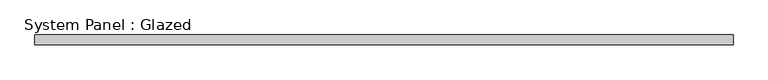
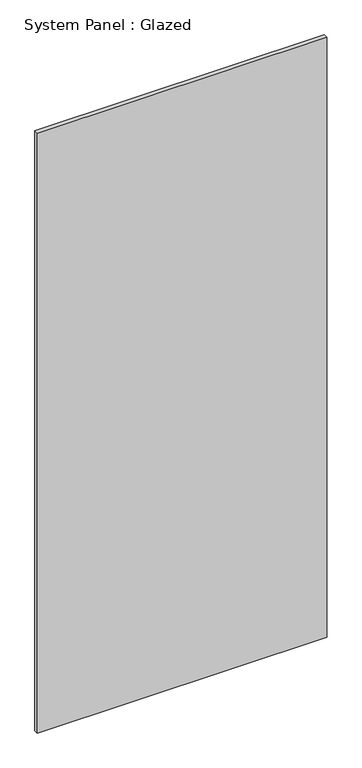
"""IFC4 building model written with IfcOpenShell, lengths in millimetres: plate geometry, System Panel : Glazed."""

import ifcopenshell
import ifcopenshell.guid

model = None  # the IFC model being written
_history = None  # IfcOwnerHistory: only IFC2X3 demands one
_inside = {}  # id of a spatial element -> (the spatial element, [elements in it])
_under = {}  # id of a project, library or spatial element -> (it, [spatial elements below it])
_declared = {}  # id of a project -> (the project, [libraries it declares])
_typed = {}  # id of a type object -> (the type object, [elements of that type])
_made_of = {}  # id of a material, layer set ... -> (it, [elements and type objects made of it])


def new_model(schema):
    """Start an empty IFC model of exactly this schema.

    Asked for "IFC4X3", IfcOpenShell would pick the latest addendum, in which some entities
    have other attributes; the version numbers below select the first issue.
    IFC2X3 requires an IfcOwnerHistory on every rooted entity: one is made here for all.
    """
    global model, _history
    if schema == "IFC4X3":
        model = ifcopenshell.file(schema_version=(4, 3, 0, 0))
    else:
        model = ifcopenshell.file(schema=schema)
    _inside.clear()
    _under.clear()
    _declared.clear()
    _typed.clear()
    _made_of.clear()
    _history = None
    if model.schema == "IFC2X3":
        org = make("IfcOrganization", Name="unknown")
        user = make(
            "IfcPersonAndOrganization",
            ThePerson=make("IfcPerson", FamilyName="unknown"),
            TheOrganization=org,
        )
        app = make(
            "IfcApplication",
            ApplicationDeveloper=org,
            Version="unknown",
            ApplicationFullName="unknown",
            ApplicationIdentifier="unknown",
        )
        _history = make(
            "IfcOwnerHistory",
            OwningUser=user,
            OwningApplication=app,
            ChangeAction="ADDED",
            CreationDate=0,
        )
    return model


def make(cls, **values):
    """One entity of the class cls with the attributes given. An attribute that is None is left unset."""
    return model.create_entity(
        cls, **{name: value for name, value in values.items() if value is not None}
    )


def rooted(cls, **values):
    """An entity with a GlobalId (a new one), such as an element, a storey or a relation."""
    return make(cls, GlobalId=ifcopenshell.guid.new(), OwnerHistory=_history, **values)


def si_unit(unit_type, name, prefix=None):
    """IfcSIUnit, for example si_unit("LENGTHUNIT", "METRE", prefix="MILLI")."""
    return make("IfcSIUnit", UnitType=unit_type, Prefix=prefix, Name=name)


def assignment(units):
    """IfcUnitAssignment: the units of a project."""
    return None if units is None else make("IfcUnitAssignment", Units=units)


def point(xyz):
    """IfcCartesianPoint."""
    return None if xyz is None else make("IfcCartesianPoint", Coordinates=xyz)


def direction(xyz):
    """IfcDirection."""
    return None if xyz is None else make("IfcDirection", DirectionRatios=xyz)


def frame(location, z_axis=None, x_axis=None):
    """IfcAxis2Placement3D, a coordinate frame: its origin and axes. An axis left out is left unset."""
    return make(
        "IfcAxis2Placement3D",
        Location=point(location),
        Axis=direction(z_axis),
        RefDirection=direction(x_axis),
    )


def origin():
    """The frame at (0, 0, 0) with its axes left unset."""
    return frame((0.0, 0.0, 0.0))


def origin_with_axes():
    """The frame at (0, 0, 0) with the z axis (0, 0, 1) and the x axis (1, 0, 0) written out."""
    return frame((0.0, 0.0, 0.0), z_axis=(0.0, 0.0, 1.0), x_axis=(1.0, 0.0, 0.0))


def place(relative_to, where):
    """IfcLocalPlacement: puts the frame where relative to a parent placement (None: the world)."""
    return make(
        "IfcLocalPlacement", PlacementRelTo=relative_to, RelativePlacement=where
    )


def context(
    kind, dimensions, precision=None, world=None, true_north=None, identifier=None
):
    """IfcGeometricRepresentationContext, for example the 3D "Model" context."""
    return make(
        "IfcGeometricRepresentationContext",
        ContextIdentifier=identifier,
        ContextType=kind,
        CoordinateSpaceDimension=dimensions,
        Precision=precision,
        WorldCoordinateSystem=world,
        TrueNorth=true_north,
    )


def project(units=None, contexts=None):
    """IfcProject with its units and contexts."""
    return rooted(
        "IfcProject",
        Name="project",
        RepresentationContexts=contexts,
        UnitsInContext=assignment(units),
    )


def spatial(cls, under=None, at=None, **own):
    """A site, building, storey or space (cls), placed at a placement, below another one or the project."""
    s = rooted(cls, ObjectPlacement=at, **own)
    if under is not None:
        _under.setdefault(under.id(), (under, []))[1].append(s)
    return s


def polyline(points):
    """IfcPolyline through the points."""
    return make("IfcPolyline", Points=[point(p) for p in points])


def outline(outer, holes=None, kind="AREA"):
    """IfcArbitraryClosedProfileDef: a profile drawn as a closed curve; with holes, ...WithVoids."""
    if holes is None:
        return make("IfcArbitraryClosedProfileDef", ProfileType=kind, OuterCurve=outer)
    return make(
        "IfcArbitraryProfileDefWithVoids",
        ProfileType=kind,
        OuterCurve=outer,
        InnerCurves=holes,
    )


def extrude(swept, where, along, depth):
    """IfcExtrudedAreaSolid: the profile swept, set in the frame where, extruded along a direction by depth."""
    return make(
        "IfcExtrudedAreaSolid",
        SweptArea=swept,
        Position=where,
        ExtrudedDirection=direction(along),
        Depth=depth,
    )


def shape(context_of_items, identifier, shape_type, items):
    """IfcShapeRepresentation: the items that make up one representation, for example the "Body"."""
    return make(
        "IfcShapeRepresentation",
        ContextOfItems=context_of_items,
        RepresentationIdentifier=identifier,
        RepresentationType=shape_type,
        Items=items,
    )


def source(mapping_origin, context_of_items, identifier, shape_type, items):
    """IfcRepresentationMap: a shape defined once, which mapped items show again and again."""
    return make(
        "IfcRepresentationMap",
        MappingOrigin=mapping_origin,
        MappedRepresentation=shape(context_of_items, identifier, shape_type, items),
    )


def transform(
    local_origin,
    x_axis=None,
    y_axis=None,
    z_axis=None,
    scale=None,
    scale2=None,
    scale3=None,
    uniform=True,
):
    """IfcCartesianTransformationOperator3D, or its non-uniform kind. x_axis, y_axis, z_axis: its Axis1, 2, 3."""
    if uniform:
        return make(
            "IfcCartesianTransformationOperator3D",
            Axis1=direction(x_axis),
            Axis2=direction(y_axis),
            LocalOrigin=point(local_origin),
            Scale=scale,
            Axis3=direction(z_axis),
        )
    return make(
        "IfcCartesianTransformationOperator3DnonUniform",
        Axis1=direction(x_axis),
        Axis2=direction(y_axis),
        LocalOrigin=point(local_origin),
        Scale=scale,
        Axis3=direction(z_axis),
        Scale2=scale2,
        Scale3=scale3,
    )


def mapped(mapping_source, mapping_target):
    """IfcMappedItem: shows the shape of a source again, moved by a transform."""
    return make(
        "IfcMappedItem", MappingSource=mapping_source, MappingTarget=mapping_target
    )


def made_of(thing, what):
    """Note that an element or type object is made of a material, layer set ...; save() writes the relation."""
    if what is not None:
        _made_of.setdefault(what.id(), (what, []))[1].append(thing)
    return thing


def element(
    cls,
    number,
    at=None,
    inside=None,
    cuts=None,
    type_object=None,
    material=None,
    context=None,
    identifier="Body",
    shape_type=None,
    held_by="IfcProductDefinitionShape",
    body=None,
    shapes=None,
    **own,
):
    """One element of the class cls, such as IfcWall. Its Tag is "e" and its number.

    at: its placement. inside: the storey or other place that contains it. cuts: it is an
    opening in that element (IfcRelVoidsElement). A single representation is given by context,
    identifier, shape_type and body (its items); several are given by shapes. held_by: the class
    of the entity that holds the representations. save() writes the other relations.
    """
    e = rooted(cls, Tag="e%d" % number, ObjectPlacement=at, **own)
    if body is not None:
        shapes = [shape(context, identifier, shape_type, body)]
    if shapes is not None:
        e.Representation = make(held_by, Representations=shapes)
    if inside is not None:
        _inside.setdefault(inside.id(), (inside, []))[1].append(e)
    if cuts is not None:
        rooted(
            "IfcRelVoidsElement", RelatingBuildingElement=cuts, RelatedOpeningElement=e
        )
    if type_object is not None:
        _typed.setdefault(type_object.id(), (type_object, []))[1].append(e)
    return made_of(e, material)


def aggregate(whole, parts):
    """IfcRelAggregates: a whole, such as a stair, and the parts it consists of."""
    return rooted("IfcRelAggregates", RelatingObject=whole, RelatedObjects=parts)


def save(model, path):
    """Write the relations noted so far, then the file.

    IfcRelAggregates (storeys below a building ...), IfcRelContainedInSpatialStructure (elements
    in a storey), IfcRelDefinesByType, IfcRelAssociatesMaterial and IfcRelDeclares: one each for
    every whole, place, type object, material and project.
    """
    for whole, parts in _under.values():
        aggregate(whole, parts)
    for where, things in _inside.values():
        rooted(
            "IfcRelContainedInSpatialStructure",
            RelatedElements=things,
            RelatingStructure=where,
        )
    for kind, things in _typed.values():
        rooted("IfcRelDefinesByType", RelatedObjects=things, RelatingType=kind)
    for what, things in _made_of.values():
        rooted("IfcRelAssociatesMaterial", RelatedObjects=things, RelatingMaterial=what)
    for by, libraries in _declared.values():
        rooted("IfcRelDeclares", RelatingContext=by, RelatedDefinitions=libraries)
    model.write(path)


def system_panel_glazed_26169dd8(model_context):
    return source(origin(), model_context, "Body", "SweptSolid", [
        extrude(outline(polyline([(890.0, 24.5), (-890.0, 24.5), (-890.0, 49.5), (890.0, 49.5), (890.0, 24.5)])), origin_with_axes(), (0.0, 0.0, 1.0), 3900.0),
    ])


if __name__ == "__main__":
    model = new_model("IFC4")
    model_context = context("Model", 3, world=origin())
    ifc_project = project(units=[si_unit("LENGTHUNIT", "METRE", prefix="MILLI")], contexts=[model_context])
    site = spatial("IfcSite", under=ifc_project)
    building = spatial("IfcBuilding", under=site)
    placement = place(None, origin())
    system_panel_glazed_shape = system_panel_glazed_26169dd8(model_context)
    element("IfcPlate", 1, ObjectType="System Panel : Glazed", at=placement, inside=building, context=model_context, shape_type="MappedRepresentation", body=[
        mapped(system_panel_glazed_shape, transform((0.0, 0.0, 0.0), x_axis=(1.0, 0.0, 0.0), y_axis=(0.0, 1.0, 0.0), z_axis=(0.0, 0.0, 1.0))),
    ])
    save(model, "model.ifc")

# Revit data of these elements
# Type "System Panel : Glazed"
#   Keynote = "H11"
#   Construction Type Id = "GSP4R"
#   Analytic Construction = "1/8 in Pilkington single glazing"
#   Visual Light Transmittance = 0.9
#   Solar Heat Gain Coefficient = 0.86
#   Heat Transfer Coefficient (U) = 6.7069 W/(m²·K)
#   Define Thermal Properties by = 1
# Element 1 (IfcPlate, "System Panel : Glazed")
#   Materials on its faces: "Glass"
# Materials
#   "Glass": class "Glass", colour RGB 0 128 192, transparency 0.9, Description = "Soda Lime Glass", Cost = 0
